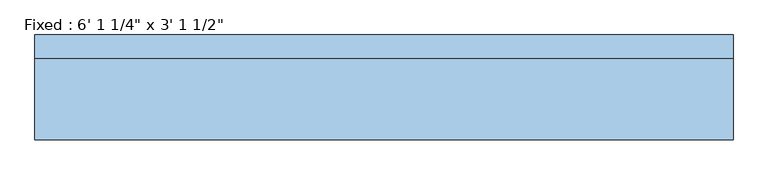
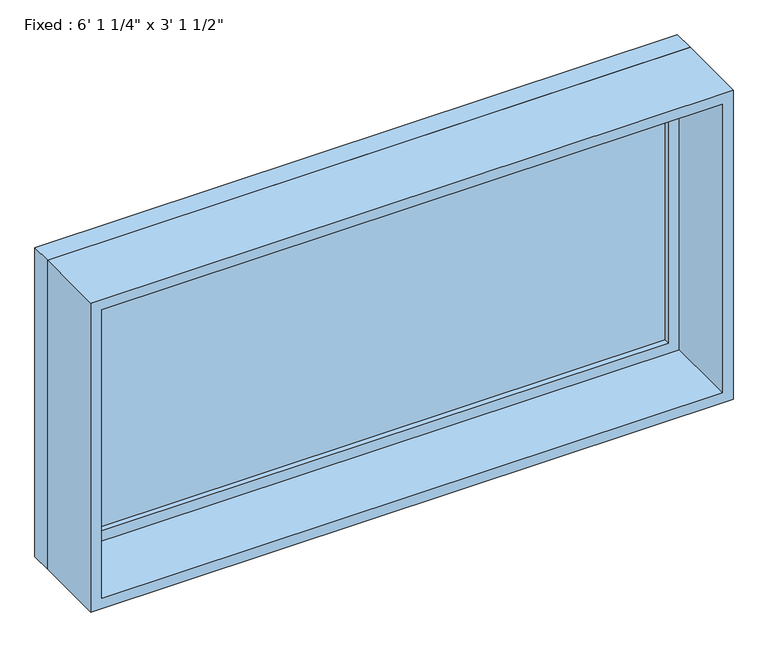
"""IFC4 building model written with IfcOpenShell, lengths in millimetres: window geometry."""

from ifc_helpers import new_model, si_unit, frame, origin, place, context, project, spatial, polyline, outline, extrude, source, transform, mapped, element, save


def window_d41c44e1(model_context):
    return source(origin(), model_context, "Body", "SweptSolid", [
        extrude(outline(polyline([(828.675, 92.075), (-904.875, 92.075), (-904.875, 104.775), (828.675, 104.775), (828.675, 92.075)])), frame((0.0, 0.0, 1257.3), z_axis=(0.0, 0.0, 1.0), x_axis=(1.0, 0.0, 0.0)), (0.0, 0.0, 1.0), 819.15),
        extrude(outline(polyline([(2120.9, -949.325), (1212.85, -949.325), (1212.85, 873.125), (2120.9, 873.125), (2120.9, -949.325)]), holes=[polyline([(2076.45, -904.875), (2076.45, 828.675), (1257.3, 828.675), (1257.3, -904.875), (2076.45, -904.875)])]), frame((0.0, 76.2, 0.0), z_axis=(0.0, 1.0, 0.0), x_axis=(0.0, 0.0, 1.0)), (0.0, 0.0, 1.0), 44.45),
        extrude(outline(polyline([(2139.95, -968.375), (1193.8, -968.375), (1193.8, 892.175), (2139.95, 892.175), (2139.95, -968.375)]), holes=[polyline([(2108.2, -936.625), (2108.2, 860.425), (1225.55, 860.425), (1225.55, -936.625), (2108.2, -936.625)])]), frame((0.0, -139.7, 0.0), z_axis=(0.0, 1.0, 0.0), x_axis=(0.0, 0.0, 1.0)), (0.0, 0.0, 1.0), 215.9),
        extrude(outline(polyline([(2139.95, 892.175), (2139.95, -968.375), (1193.8, -968.375), (1193.8, 892.175), (2139.95, 892.175)]), holes=[polyline([(2120.9, 873.125), (1212.85, 873.125), (1212.85, -949.325), (2120.9, -949.325), (2120.9, 873.125)])]), frame((0.0, 76.2, 0.0), z_axis=(0.0, 1.0, 0.0), x_axis=(0.0, 0.0, 1.0)), (0.0, 0.0, 1.0), 63.5),
    ])


if __name__ == "__main__":
    model = new_model("IFC4")
    model_context = context("Model", 3, world=origin())
    ifc_project = project(units=[si_unit("LENGTHUNIT", "METRE", prefix="MILLI")], contexts=[model_context])
    site = spatial("IfcSite", under=ifc_project)
    building = spatial("IfcBuilding", under=site)
    placement = place(None, origin())
    window_shape = window_d41c44e1(model_context)
    element("IfcWindow", 1, ObjectType="Fixed : 6' 1 1/4\" x 3' 1 1/2\"", at=placement, inside=building, context=model_context, shape_type="MappedRepresentation", body=[
        mapped(window_shape, transform((0.0, 0.0, 0.0), x_axis=(1.0, 0.0, 0.0), y_axis=(0.0, 1.0, 0.0), z_axis=(0.0, 0.0, 1.0))),
    ])
    save(model, "model.ifc")

# Revit data of these elements
# Type "Fixed : 6' 1 1/4\" x 3' 1 1/2\""
#   Type Mark = "21"
#   Assembly Code = "B2020100"
#   Height = 3' - 1 1/4"
#   Default Sill Height = 3' - 11"
#   Width = 6' - 1 1/4"
#   Window Inset = 0' - 0 3/4"
#   Glass Pane Material = Glass
#   Sash Material = accent 2
#   Wall Closure = (empty or 0)
# Element 1 (IfcWindow, "Fixed : 6' 1 1/4\" x 3' 1 1/2\"")
#   Materials on its faces: "accent 2", "Glass"
# Materials
#   "Glass": class "Glass", colour RGB 236 240 239, transparency 0.85, Description = "Soda Lime Glass", Cost = 0
#   "accent 2": class "Wood", colour RGB 80 80 80, transparency 0, Description = "Wood framing, thermal airspace", Cost = 0
